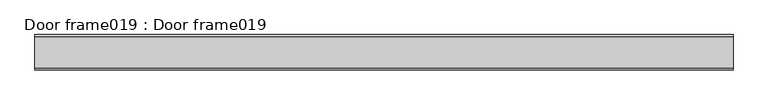
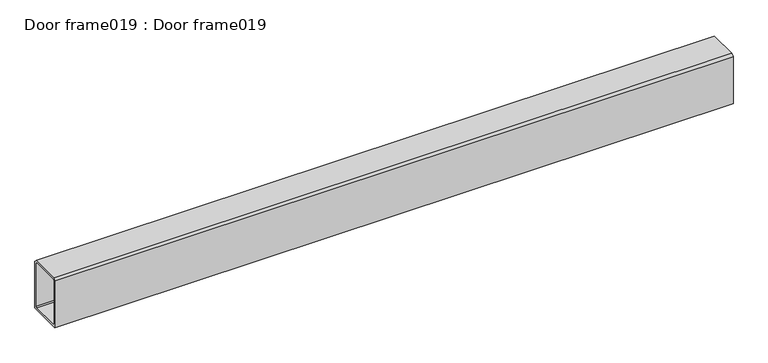
"""IFC4 building model written with IfcOpenShell, lengths in millimetres: proxy geometry, Door frame019 : Door frame019."""

from ifc_helpers import new_model, si_unit, frame, origin, place, context, project, spatial, polyline, outline, extrude, source, transform, mapped, element, save


def door_frame019_door_frame019_9a35ada2(model_context):
    return source(origin(), model_context, "Body", "SweptSolid", [
        extrude(outline(polyline([(9744.174946, 39528.496), (9750.524946, 39522.146), (9750.524946, 39376.096), (9648.924946, 39376.096), (9648.924946, 39522.146), (9655.274946, 39528.496), (9744.174946, 39528.496)]), holes=[polyline([(9744.174946, 39385.0762561), (9744.174946, 39519.5157439), (9741.5446899, 39522.146), (9657.9052021, 39522.146), (9655.274946, 39519.5157439), (9655.274946, 39385.0762561), (9657.9052021, 39382.446), (9741.5446899, 39382.446), (9744.174946, 39385.0762561)])]), frame((-9232.0719278, 0.0, 0.0), z_axis=(1.0, 0.0, 0.0), x_axis=(0.0, 1.0, 0.0)), (0.0, 0.0, 1.0), 1999.85),
    ])


if __name__ == "__main__":
    model = new_model("IFC4")
    model_context = context("Model", 3, world=origin())
    ifc_project = project(units=[si_unit("LENGTHUNIT", "METRE", prefix="MILLI")], contexts=[model_context])
    site = spatial("IfcSite", under=ifc_project)
    building = spatial("IfcBuilding", under=site)
    placement = place(None, origin())
    door_frame019_door_frame019_shape = door_frame019_door_frame019_9a35ada2(model_context)
    element("IfcBuildingElementProxy", 1, Name="Door frame019 : Door frame019", ObjectType="Door frame019 : Door frame019", at=placement, inside=building, context=model_context, shape_type="MappedRepresentation", body=[
        mapped(door_frame019_door_frame019_shape, transform((0.0, 0.0, 0.0), x_axis=(1.0, 0.0, 0.0), y_axis=(0.0, 1.0, 0.0), z_axis=(0.0, 0.0, 1.0))),
    ])
    save(model, "model.ifc")

# Revit data of these elements
# Type "Door frame019 : Door frame019"
#   NameOverride = "Door frame019"
# Element 1 (IfcBuildingElementProxy, "Door frame019 : Door frame019")
#   Materials on its faces: "DOOR FRAME: TUBE STEEL PROFILE - METALIZED, PRIMED & PAINTED (COLOR PER ARCHITECT)"
# Materials
#   "DOOR FRAME: TUBE STEEL PROFILE - METALIZED, PRIMED & PAINTED (COLOR PER ARCHITECT)": class "Unassigned", colour RGB 128 128 128, transparency 0, Cost = 0
